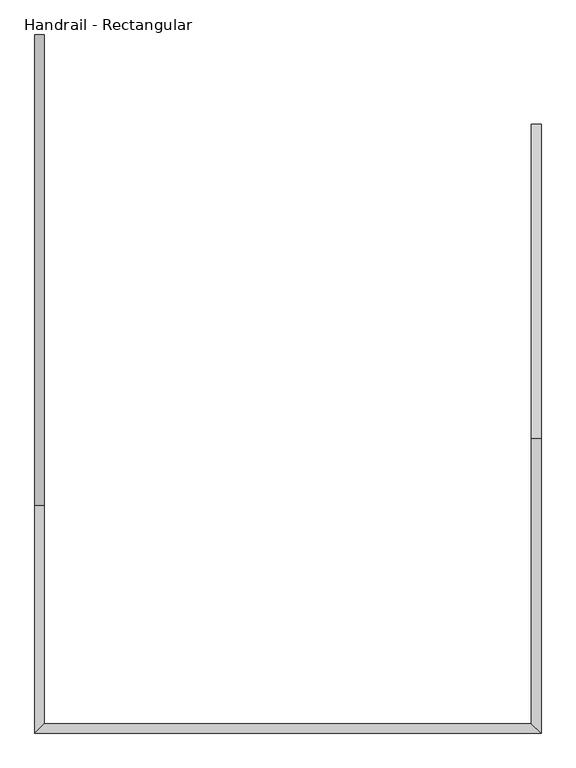
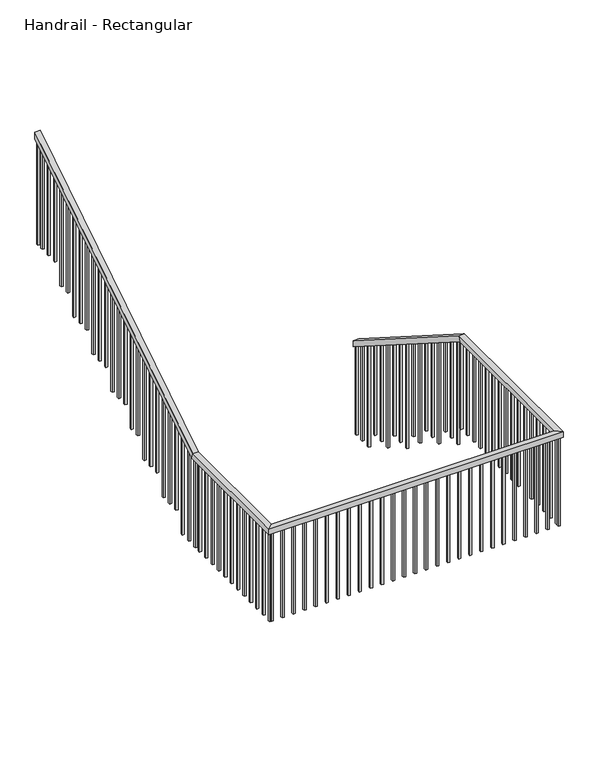
"""IFC4 building model written with IfcOpenShell, lengths in millimetres: railing geometry, Handrail - Rectangular."""

from ifc_helpers import new_model, si_unit, frame, origin, place, context, project, spatial, polyline, outline, extrude, faceted_brep, source, transform, mapped, element, save


def handrail_rectangular_a87038dc(model_context):
    return source(origin(), model_context, "Body", "SolidModel", [
        faceted_brep([(-73285.35, 12128.5, 20345.4), (-73285.35, 12128.5, 20285.186276), (-73336.15, 12128.5, 20285.186276), (-73336.15, 12128.5, 20345.4), (-73285.35, 10452.1, 21412.2), (-73285.35, 10437.3070051, 21361.4), (-73336.15, 10437.3070051, 21361.4), (-73336.15, 10452.1, 21412.2), (-73285.35, 8877.3, 21412.2), (-73285.35, 8877.3, 21361.4), (-73336.15, 8928.1, 21361.4), (-73336.15, 8928.1, 21412.2), (-75990.45, 8877.3, 21412.2), (-75990.45, 8877.3, 21361.4), (-75939.65, 8928.1, 21361.4), (-75939.65, 8928.1, 21412.2), (-75990.45, 10090.15, 21412.2), (-75990.45, 10104.9429949, 21361.4), (-75939.65, 10104.9429949, 21361.4), (-75939.65, 10090.15, 21412.2), (-75990.45, 12604.75, 23012.4), (-75939.65, 12604.75, 23012.4), (-75939.65, 12604.75, 22952.186276), (-75990.45, 12604.75, 22952.186276)], [[[0, 1, 2, 3]], [[1, 0, 4, 5]], [[2, 1, 5, 6]], [[3, 2, 6, 7]], [[0, 3, 7, 4]], [[5, 4, 8, 9]], [[6, 5, 9, 10]], [[7, 6, 10, 11]], [[4, 7, 11, 8]], [[9, 8, 12, 13]], [[10, 9, 13, 14]], [[11, 10, 14, 15]], [[8, 11, 15, 12]], [[13, 12, 16, 17]], [[14, 13, 17, 18]], [[15, 14, 18, 19]], [[12, 15, 19, 16]], [[20, 21, 22, 23]], [[17, 16, 20, 23]], [[18, 17, 23, 22]], [[19, 18, 22, 21]], [[16, 19, 21, 20]]]),
        extrude(outline(polyline([(12538.075, 22909.7567305), (12538.075, 21920.2), (12519.025, 21920.2), (12519.025, 22897.6340032), (12538.075, 22909.7567305)])), frame((-75974.575, 0.0, 0.0), z_axis=(1.0, 0.0, 0.0), x_axis=(0.0, 1.0, 0.0)), (0.0, 0.0, 1.0), 19.05),
        extrude(outline(polyline([(12436.475, 22845.1021851), (12436.475, 21920.2), (12417.425, 21920.2), (12417.425, 22832.9794578), (12436.475, 22845.1021851)])), frame((-75974.575, 0.0, 0.0), z_axis=(1.0, 0.0, 0.0), x_axis=(0.0, 1.0, 0.0)), (0.0, 0.0, 1.0), 19.05),
        extrude(outline(polyline([(12334.875, 22780.4476396), (12334.875, 21920.2), (12315.825, 21920.2), (12315.825, 22768.3249123), (12334.875, 22780.4476396)])), frame((-75974.575, 0.0, 0.0), z_axis=(1.0, 0.0, 0.0), x_axis=(0.0, 1.0, 0.0)), (0.0, 0.0, 1.0), 19.05),
        extrude(outline(polyline([(12233.275, 22715.7930941), (12233.275, 21742.4), (12214.225, 21742.4), (12214.225, 22703.6703669), (12233.275, 22715.7930941)])), frame((-75974.575, 0.0, 0.0), z_axis=(1.0, 0.0, 0.0), x_axis=(0.0, 1.0, 0.0)), (0.0, 0.0, 1.0), 19.05),
        extrude(outline(polyline([(12131.675, 22651.1385487), (12131.675, 21742.4), (12112.625, 21742.4), (12112.625, 22639.0158214), (12131.675, 22651.1385487)])), frame((-75974.575, 0.0, 0.0), z_axis=(1.0, 0.0, 0.0), x_axis=(0.0, 1.0, 0.0)), (0.0, 0.0, 1.0), 19.05),
        extrude(outline(polyline([(12030.075, 22586.4840032), (12030.075, 21564.6), (12011.025, 21564.6), (12011.025, 22574.361276), (12030.075, 22586.4840032)])), frame((-75974.575, 0.0, 0.0), z_axis=(1.0, 0.0, 0.0), x_axis=(0.0, 1.0, 0.0)), (0.0, 0.0, 1.0), 19.05),
        extrude(outline(polyline([(11928.475, 22521.8294578), (11928.475, 21564.6), (11909.425, 21564.6), (11909.425, 22509.7067305), (11928.475, 22521.8294578)])), frame((-75974.575, 0.0, 0.0), z_axis=(1.0, 0.0, 0.0), x_axis=(0.0, 1.0, 0.0)), (0.0, 0.0, 1.0), 19.05),
        extrude(outline(polyline([(11826.875, 22457.1749123), (11826.875, 21564.6), (11807.825, 21564.6), (11807.825, 22445.0521851), (11826.875, 22457.1749123)])), frame((-75974.575, 0.0, 0.0), z_axis=(1.0, 0.0, 0.0), x_axis=(0.0, 1.0, 0.0)), (0.0, 0.0, 1.0), 19.05),
        extrude(outline(polyline([(11725.275, 22392.5203669), (11725.275, 21386.8), (11706.225, 21386.8), (11706.225, 22380.3976396), (11725.275, 22392.5203669)])), frame((-75974.575, 0.0, 0.0), z_axis=(1.0, 0.0, 0.0), x_axis=(0.0, 1.0, 0.0)), (0.0, 0.0, 1.0), 19.05),
        extrude(outline(polyline([(11623.675, 22327.8658214), (11623.675, 21386.8), (11604.625, 21386.8), (11604.625, 22315.7430941), (11623.675, 22327.8658214)])), frame((-75974.575, 0.0, 0.0), z_axis=(1.0, 0.0, 0.0), x_axis=(0.0, 1.0, 0.0)), (0.0, 0.0, 1.0), 19.05),
        extrude(outline(polyline([(11522.075, 22263.211276), (11522.075, 21386.8), (11503.025, 21386.8), (11503.025, 22251.0885487), (11522.075, 22263.211276)])), frame((-75974.575, 0.0, 0.0), z_axis=(1.0, 0.0, 0.0), x_axis=(0.0, 1.0, 0.0)), (0.0, 0.0, 1.0), 19.05),
        extrude(outline(polyline([(11420.475, 22198.5567305), (11420.475, 21209.0), (11401.425, 21209.0), (11401.425, 22186.4340032), (11420.475, 22198.5567305)])), frame((-75974.575, 0.0, 0.0), z_axis=(1.0, 0.0, 0.0), x_axis=(0.0, 1.0, 0.0)), (0.0, 0.0, 1.0), 19.05),
        extrude(outline(polyline([(11318.875, 22133.9021851), (11318.875, 21209.0), (11299.825, 21209.0), (11299.825, 22121.7794578), (11318.875, 22133.9021851)])), frame((-75974.575, 0.0, 0.0), z_axis=(1.0, 0.0, 0.0), x_axis=(0.0, 1.0, 0.0)), (0.0, 0.0, 1.0), 19.05),
        extrude(outline(polyline([(11217.275, 22069.2476396), (11217.275, 21209.0), (11198.225, 21209.0), (11198.225, 22057.1249123), (11217.275, 22069.2476396)])), frame((-75974.575, 0.0, 0.0), z_axis=(1.0, 0.0, 0.0), x_axis=(0.0, 1.0, 0.0)), (0.0, 0.0, 1.0), 19.05),
        extrude(outline(polyline([(11115.675, 22004.5930941), (11115.675, 21031.2), (11096.625, 21031.2), (11096.625, 21992.4703669), (11115.675, 22004.5930941)])), frame((-75974.575, 0.0, 0.0), z_axis=(1.0, 0.0, 0.0), x_axis=(0.0, 1.0, 0.0)), (0.0, 0.0, 1.0), 19.05),
        extrude(outline(polyline([(11014.075, 21939.9385487), (11014.075, 21031.2), (10995.025, 21031.2), (10995.025, 21927.8158214), (11014.075, 21939.9385487)])), frame((-75974.575, 0.0, 0.0), z_axis=(1.0, 0.0, 0.0), x_axis=(0.0, 1.0, 0.0)), (0.0, 0.0, 1.0), 19.05),
        extrude(outline(polyline([(10912.475, 21875.2840032), (10912.475, 20853.4), (10893.425, 20853.4), (10893.425, 21863.161276), (10912.475, 21875.2840032)])), frame((-75974.575, 0.0, 0.0), z_axis=(1.0, 0.0, 0.0), x_axis=(0.0, 1.0, 0.0)), (0.0, 0.0, 1.0), 19.05),
        extrude(outline(polyline([(10810.875, 21810.6294578), (10810.875, 20853.4), (10791.825, 20853.4), (10791.825, 21798.5067305), (10810.875, 21810.6294578)])), frame((-75974.575, 0.0, 0.0), z_axis=(1.0, 0.0, 0.0), x_axis=(0.0, 1.0, 0.0)), (0.0, 0.0, 1.0), 19.05),
        extrude(outline(polyline([(10709.275, 21745.9749123), (10709.275, 20853.4), (10690.225, 20853.4), (10690.225, 21733.8521851), (10709.275, 21745.9749123)])), frame((-75974.575, 0.0, 0.0), z_axis=(1.0, 0.0, 0.0), x_axis=(0.0, 1.0, 0.0)), (0.0, 0.0, 1.0), 19.05),
        extrude(outline(polyline([(10607.675, 21681.3203669), (10607.675, 20675.6), (10588.625, 20675.6), (10588.625, 21669.1976396), (10607.675, 21681.3203669)])), frame((-75974.575, 0.0, 0.0), z_axis=(1.0, 0.0, 0.0), x_axis=(0.0, 1.0, 0.0)), (0.0, 0.0, 1.0), 19.05),
        extrude(outline(polyline([(10506.075, 21616.6658214), (10506.075, 20675.6), (10487.025, 20675.6), (10487.025, 21604.5430941), (10506.075, 21616.6658214)])), frame((-75974.575, 0.0, 0.0), z_axis=(1.0, 0.0, 0.0), x_axis=(0.0, 1.0, 0.0)), (0.0, 0.0, 1.0), 19.05),
        extrude(outline(polyline([(10404.475, 21552.011276), (10404.475, 20675.6), (10385.425, 20675.6), (10385.425, 21539.8885487), (10404.475, 21552.011276)])), frame((-75974.575, 0.0, 0.0), z_axis=(1.0, 0.0, 0.0), x_axis=(0.0, 1.0, 0.0)), (0.0, 0.0, 1.0), 19.05),
        extrude(outline(polyline([(10302.875, 21487.3567305), (10302.875, 20497.8), (10283.825, 20497.8), (10283.825, 21475.2340032), (10302.875, 21487.3567305)])), frame((-75974.575, 0.0, 0.0), z_axis=(1.0, 0.0, 0.0), x_axis=(0.0, 1.0, 0.0)), (0.0, 0.0, 1.0), 19.05),
        extrude(outline(polyline([(10201.275, 21422.7021851), (10201.275, 20497.8), (10182.225, 20497.8), (10182.225, 21410.5794578), (10201.275, 21422.7021851)])), frame((-75974.575, 0.0, 0.0), z_axis=(1.0, 0.0, 0.0), x_axis=(0.0, 1.0, 0.0)), (0.0, 0.0, 1.0), 19.05),
        extrude(outline(polyline([(-75974.575, 10010.775), (-75974.575, 10029.825), (-75955.525, 10029.825), (-75955.525, 10010.775), (-75974.575, 10010.775)])), frame((0.0, 0.0, 20497.8), z_axis=(0.0, 0.0, 1.0), x_axis=(1.0, 0.0, 0.0)), (0.0, 0.0, 1.0), 863.6),
        extrude(outline(polyline([(-75974.575, 9909.175), (-75974.575, 9928.225), (-75955.525, 9928.225), (-75955.525, 9909.175), (-75974.575, 9909.175)])), frame((0.0, 0.0, 20497.8), z_axis=(0.0, 0.0, 1.0), x_axis=(1.0, 0.0, 0.0)), (0.0, 0.0, 1.0), 863.6),
        extrude(outline(polyline([(-75974.575, 9807.575), (-75974.575, 9826.625), (-75955.525, 9826.625), (-75955.525, 9807.575), (-75974.575, 9807.575)])), frame((0.0, 0.0, 20497.8), z_axis=(0.0, 0.0, 1.0), x_axis=(1.0, 0.0, 0.0)), (0.0, 0.0, 1.0), 863.6),
        extrude(outline(polyline([(-75974.575, 9705.975), (-75974.575, 9725.025), (-75955.525, 9725.025), (-75955.525, 9705.975), (-75974.575, 9705.975)])), frame((0.0, 0.0, 20497.8), z_axis=(0.0, 0.0, 1.0), x_axis=(1.0, 0.0, 0.0)), (0.0, 0.0, 1.0), 863.6),
        extrude(outline(polyline([(-75974.575, 9604.375), (-75974.575, 9623.425), (-75955.525, 9623.425), (-75955.525, 9604.375), (-75974.575, 9604.375)])), frame((0.0, 0.0, 20497.8), z_axis=(0.0, 0.0, 1.0), x_axis=(1.0, 0.0, 0.0)), (0.0, 0.0, 1.0), 863.6),
        extrude(outline(polyline([(-75974.575, 9502.775), (-75974.575, 9521.825), (-75955.525, 9521.825), (-75955.525, 9502.775), (-75974.575, 9502.775)])), frame((0.0, 0.0, 20497.8), z_axis=(0.0, 0.0, 1.0), x_axis=(1.0, 0.0, 0.0)), (0.0, 0.0, 1.0), 863.6),
        extrude(outline(polyline([(-75974.575, 9401.175), (-75974.575, 9420.225), (-75955.525, 9420.225), (-75955.525, 9401.175), (-75974.575, 9401.175)])), frame((0.0, 0.0, 20497.8), z_axis=(0.0, 0.0, 1.0), x_axis=(1.0, 0.0, 0.0)), (0.0, 0.0, 1.0), 863.6),
        extrude(outline(polyline([(-75974.575, 9299.575), (-75974.575, 9318.625), (-75955.525, 9318.625), (-75955.525, 9299.575), (-75974.575, 9299.575)])), frame((0.0, 0.0, 20497.8), z_axis=(0.0, 0.0, 1.0), x_axis=(1.0, 0.0, 0.0)), (0.0, 0.0, 1.0), 863.6),
        extrude(outline(polyline([(-75974.575, 9197.975), (-75974.575, 9217.025), (-75955.525, 9217.025), (-75955.525, 9197.975), (-75974.575, 9197.975)])), frame((0.0, 0.0, 20497.8), z_axis=(0.0, 0.0, 1.0), x_axis=(1.0, 0.0, 0.0)), (0.0, 0.0, 1.0), 863.6),
        extrude(outline(polyline([(-75974.575, 9096.375), (-75974.575, 9115.425), (-75955.525, 9115.425), (-75955.525, 9096.375), (-75974.575, 9096.375)])), frame((0.0, 0.0, 20497.8), z_axis=(0.0, 0.0, 1.0), x_axis=(1.0, 0.0, 0.0)), (0.0, 0.0, 1.0), 863.6),
        extrude(outline(polyline([(-75974.575, 8994.775), (-75974.575, 9013.825), (-75955.525, 9013.825), (-75955.525, 8994.775), (-75974.575, 8994.775)])), frame((0.0, 0.0, 20497.8), z_axis=(0.0, 0.0, 1.0), x_axis=(1.0, 0.0, 0.0)), (0.0, 0.0, 1.0), 863.6),
        extrude(outline(polyline([(-75942.825, 8893.175), (-75961.875, 8893.175), (-75961.875, 8912.225), (-75942.825, 8912.225), (-75942.825, 8893.175)])), frame((0.0, 0.0, 20497.8), z_axis=(0.0, 0.0, 1.0), x_axis=(1.0, 0.0, 0.0)), (0.0, 0.0, 1.0), 863.6),
        extrude(outline(polyline([(-75841.225, 8893.175), (-75860.275, 8893.175), (-75860.275, 8912.225), (-75841.225, 8912.225), (-75841.225, 8893.175)])), frame((0.0, 0.0, 20497.8), z_axis=(0.0, 0.0, 1.0), x_axis=(1.0, 0.0, 0.0)), (0.0, 0.0, 1.0), 863.6),
        extrude(outline(polyline([(-75739.625, 8893.175), (-75758.675, 8893.175), (-75758.675, 8912.225), (-75739.625, 8912.225), (-75739.625, 8893.175)])), frame((0.0, 0.0, 20497.8), z_axis=(0.0, 0.0, 1.0), x_axis=(1.0, 0.0, 0.0)), (0.0, 0.0, 1.0), 863.6),
        extrude(outline(polyline([(-75638.025, 8893.175), (-75657.075, 8893.175), (-75657.075, 8912.225), (-75638.025, 8912.225), (-75638.025, 8893.175)])), frame((0.0, 0.0, 20497.8), z_axis=(0.0, 0.0, 1.0), x_axis=(1.0, 0.0, 0.0)), (0.0, 0.0, 1.0), 863.6),
        extrude(outline(polyline([(-75536.425, 8893.175), (-75555.475, 8893.175), (-75555.475, 8912.225), (-75536.425, 8912.225), (-75536.425, 8893.175)])), frame((0.0, 0.0, 20497.8), z_axis=(0.0, 0.0, 1.0), x_axis=(1.0, 0.0, 0.0)), (0.0, 0.0, 1.0), 863.6),
        extrude(outline(polyline([(-75434.825, 8893.175), (-75453.875, 8893.175), (-75453.875, 8912.225), (-75434.825, 8912.225), (-75434.825, 8893.175)])), frame((0.0, 0.0, 20497.8), z_axis=(0.0, 0.0, 1.0), x_axis=(1.0, 0.0, 0.0)), (0.0, 0.0, 1.0), 863.6),
        extrude(outline(polyline([(-75333.225, 8893.175), (-75352.275, 8893.175), (-75352.275, 8912.225), (-75333.225, 8912.225), (-75333.225, 8893.175)])), frame((0.0, 0.0, 20497.8), z_axis=(0.0, 0.0, 1.0), x_axis=(1.0, 0.0, 0.0)), (0.0, 0.0, 1.0), 863.6),
        extrude(outline(polyline([(-75231.625, 8893.175), (-75250.675, 8893.175), (-75250.675, 8912.225), (-75231.625, 8912.225), (-75231.625, 8893.175)])), frame((0.0, 0.0, 20497.8), z_axis=(0.0, 0.0, 1.0), x_axis=(1.0, 0.0, 0.0)), (0.0, 0.0, 1.0), 863.6),
        extrude(outline(polyline([(-75130.025, 8893.175), (-75149.075, 8893.175), (-75149.075, 8912.225), (-75130.025, 8912.225), (-75130.025, 8893.175)])), frame((0.0, 0.0, 20497.8), z_axis=(0.0, 0.0, 1.0), x_axis=(1.0, 0.0, 0.0)), (0.0, 0.0, 1.0), 863.6),
        extrude(outline(polyline([(-75028.425, 8893.175), (-75047.475, 8893.175), (-75047.475, 8912.225), (-75028.425, 8912.225), (-75028.425, 8893.175)])), frame((0.0, 0.0, 20497.8), z_axis=(0.0, 0.0, 1.0), x_axis=(1.0, 0.0, 0.0)), (0.0, 0.0, 1.0), 863.6),
        extrude(outline(polyline([(-74926.825, 8893.175), (-74945.875, 8893.175), (-74945.875, 8912.225), (-74926.825, 8912.225), (-74926.825, 8893.175)])), frame((0.0, 0.0, 20497.8), z_axis=(0.0, 0.0, 1.0), x_axis=(1.0, 0.0, 0.0)), (0.0, 0.0, 1.0), 863.6),
        extrude(outline(polyline([(-74825.225, 8893.175), (-74844.275, 8893.175), (-74844.275, 8912.225), (-74825.225, 8912.225), (-74825.225, 8893.175)])), frame((0.0, 0.0, 20497.8), z_axis=(0.0, 0.0, 1.0), x_axis=(1.0, 0.0, 0.0)), (0.0, 0.0, 1.0), 863.6),
        extrude(outline(polyline([(-74723.625, 8893.175), (-74742.675, 8893.175), (-74742.675, 8912.225), (-74723.625, 8912.225), (-74723.625, 8893.175)])), frame((0.0, 0.0, 20497.8), z_axis=(0.0, 0.0, 1.0), x_axis=(1.0, 0.0, 0.0)), (0.0, 0.0, 1.0), 863.6),
        extrude(outline(polyline([(-74622.025, 8893.175), (-74641.075, 8893.175), (-74641.075, 8912.225), (-74622.025, 8912.225), (-74622.025, 8893.175)])), frame((0.0, 0.0, 20497.8), z_axis=(0.0, 0.0, 1.0), x_axis=(1.0, 0.0, 0.0)), (0.0, 0.0, 1.0), 863.6),
        extrude(outline(polyline([(-74520.425, 8893.175), (-74539.475, 8893.175), (-74539.475, 8912.225), (-74520.425, 8912.225), (-74520.425, 8893.175)])), frame((0.0, 0.0, 20497.8), z_axis=(0.0, 0.0, 1.0), x_axis=(1.0, 0.0, 0.0)), (0.0, 0.0, 1.0), 863.6),
        extrude(outline(polyline([(-74418.825, 8893.175), (-74437.875, 8893.175), (-74437.875, 8912.225), (-74418.825, 8912.225), (-74418.825, 8893.175)])), frame((0.0, 0.0, 20497.8), z_axis=(0.0, 0.0, 1.0), x_axis=(1.0, 0.0, 0.0)), (0.0, 0.0, 1.0), 863.6),
        extrude(outline(polyline([(-74317.225, 8893.175), (-74336.275, 8893.175), (-74336.275, 8912.225), (-74317.225, 8912.225), (-74317.225, 8893.175)])), frame((0.0, 0.0, 20497.8), z_axis=(0.0, 0.0, 1.0), x_axis=(1.0, 0.0, 0.0)), (0.0, 0.0, 1.0), 863.6),
        extrude(outline(polyline([(-74215.625, 8893.175), (-74234.675, 8893.175), (-74234.675, 8912.225), (-74215.625, 8912.225), (-74215.625, 8893.175)])), frame((0.0, 0.0, 20497.8), z_axis=(0.0, 0.0, 1.0), x_axis=(1.0, 0.0, 0.0)), (0.0, 0.0, 1.0), 863.6),
        extrude(outline(polyline([(-74114.025, 8893.175), (-74133.075, 8893.175), (-74133.075, 8912.225), (-74114.025, 8912.225), (-74114.025, 8893.175)])), frame((0.0, 0.0, 20497.8), z_axis=(0.0, 0.0, 1.0), x_axis=(1.0, 0.0, 0.0)), (0.0, 0.0, 1.0), 863.6),
        extrude(outline(polyline([(-74012.425, 8893.175), (-74031.475, 8893.175), (-74031.475, 8912.225), (-74012.425, 8912.225), (-74012.425, 8893.175)])), frame((0.0, 0.0, 20497.8), z_axis=(0.0, 0.0, 1.0), x_axis=(1.0, 0.0, 0.0)), (0.0, 0.0, 1.0), 863.6),
        extrude(outline(polyline([(-73910.825, 8893.175), (-73929.875, 8893.175), (-73929.875, 8912.225), (-73910.825, 8912.225), (-73910.825, 8893.175)])), frame((0.0, 0.0, 20497.8), z_axis=(0.0, 0.0, 1.0), x_axis=(1.0, 0.0, 0.0)), (0.0, 0.0, 1.0), 863.6),
        extrude(outline(polyline([(-73809.225, 8893.175), (-73828.275, 8893.175), (-73828.275, 8912.225), (-73809.225, 8912.225), (-73809.225, 8893.175)])), frame((0.0, 0.0, 20497.8), z_axis=(0.0, 0.0, 1.0), x_axis=(1.0, 0.0, 0.0)), (0.0, 0.0, 1.0), 863.6),
        extrude(outline(polyline([(-73707.625, 8893.175), (-73726.675, 8893.175), (-73726.675, 8912.225), (-73707.625, 8912.225), (-73707.625, 8893.175)])), frame((0.0, 0.0, 20497.8), z_axis=(0.0, 0.0, 1.0), x_axis=(1.0, 0.0, 0.0)), (0.0, 0.0, 1.0), 863.6),
        extrude(outline(polyline([(-73606.025, 8893.175), (-73625.075, 8893.175), (-73625.075, 8912.225), (-73606.025, 8912.225), (-73606.025, 8893.175)])), frame((0.0, 0.0, 20497.8), z_axis=(0.0, 0.0, 1.0), x_axis=(1.0, 0.0, 0.0)), (0.0, 0.0, 1.0), 863.6),
        extrude(outline(polyline([(-73504.425, 8893.175), (-73523.475, 8893.175), (-73523.475, 8912.225), (-73504.425, 8912.225), (-73504.425, 8893.175)])), frame((0.0, 0.0, 20497.8), z_axis=(0.0, 0.0, 1.0), x_axis=(1.0, 0.0, 0.0)), (0.0, 0.0, 1.0), 863.6),
        extrude(outline(polyline([(-73402.825, 8893.175), (-73421.875, 8893.175), (-73421.875, 8912.225), (-73402.825, 8912.225), (-73402.825, 8893.175)])), frame((0.0, 0.0, 20497.8), z_axis=(0.0, 0.0, 1.0), x_axis=(1.0, 0.0, 0.0)), (0.0, 0.0, 1.0), 863.6),
        extrude(outline(polyline([(-73301.225, 8937.625), (-73301.225, 8918.575), (-73320.275, 8918.575), (-73320.275, 8937.625), (-73301.225, 8937.625)])), frame((0.0, 0.0, 20497.8), z_axis=(0.0, 0.0, 1.0), x_axis=(1.0, 0.0, 0.0)), (0.0, 0.0, 1.0), 863.6),
        extrude(outline(polyline([(-73301.225, 9039.225), (-73301.225, 9020.175), (-73320.275, 9020.175), (-73320.275, 9039.225), (-73301.225, 9039.225)])), frame((0.0, 0.0, 20497.8), z_axis=(0.0, 0.0, 1.0), x_axis=(1.0, 0.0, 0.0)), (0.0, 0.0, 1.0), 863.6),
        extrude(outline(polyline([(-73301.225, 9140.825), (-73301.225, 9121.775), (-73320.275, 9121.775), (-73320.275, 9140.825), (-73301.225, 9140.825)])), frame((0.0, 0.0, 20497.8), z_axis=(0.0, 0.0, 1.0), x_axis=(1.0, 0.0, 0.0)), (0.0, 0.0, 1.0), 863.6),
        extrude(outline(polyline([(-73301.225, 9242.425), (-73301.225, 9223.375), (-73320.275, 9223.375), (-73320.275, 9242.425), (-73301.225, 9242.425)])), frame((0.0, 0.0, 20497.8), z_axis=(0.0, 0.0, 1.0), x_axis=(1.0, 0.0, 0.0)), (0.0, 0.0, 1.0), 863.6),
        extrude(outline(polyline([(-73301.225, 9344.025), (-73301.225, 9324.975), (-73320.275, 9324.975), (-73320.275, 9344.025), (-73301.225, 9344.025)])), frame((0.0, 0.0, 20497.8), z_axis=(0.0, 0.0, 1.0), x_axis=(1.0, 0.0, 0.0)), (0.0, 0.0, 1.0), 863.6),
        extrude(outline(polyline([(-73301.225, 9445.625), (-73301.225, 9426.575), (-73320.275, 9426.575), (-73320.275, 9445.625), (-73301.225, 9445.625)])), frame((0.0, 0.0, 20497.8), z_axis=(0.0, 0.0, 1.0), x_axis=(1.0, 0.0, 0.0)), (0.0, 0.0, 1.0), 863.6),
        extrude(outline(polyline([(-73301.225, 9547.225), (-73301.225, 9528.175), (-73320.275, 9528.175), (-73320.275, 9547.225), (-73301.225, 9547.225)])), frame((0.0, 0.0, 20497.8), z_axis=(0.0, 0.0, 1.0), x_axis=(1.0, 0.0, 0.0)), (0.0, 0.0, 1.0), 863.6),
        extrude(outline(polyline([(-73301.225, 9648.825), (-73301.225, 9629.775), (-73320.275, 9629.775), (-73320.275, 9648.825), (-73301.225, 9648.825)])), frame((0.0, 0.0, 20497.8), z_axis=(0.0, 0.0, 1.0), x_axis=(1.0, 0.0, 0.0)), (0.0, 0.0, 1.0), 863.6),
        extrude(outline(polyline([(-73301.225, 9750.425), (-73301.225, 9731.375), (-73320.275, 9731.375), (-73320.275, 9750.425), (-73301.225, 9750.425)])), frame((0.0, 0.0, 20497.8), z_axis=(0.0, 0.0, 1.0), x_axis=(1.0, 0.0, 0.0)), (0.0, 0.0, 1.0), 863.6),
        extrude(outline(polyline([(-73301.225, 9852.025), (-73301.225, 9832.975), (-73320.275, 9832.975), (-73320.275, 9852.025), (-73301.225, 9852.025)])), frame((0.0, 0.0, 20497.8), z_axis=(0.0, 0.0, 1.0), x_axis=(1.0, 0.0, 0.0)), (0.0, 0.0, 1.0), 863.6),
        extrude(outline(polyline([(-73301.225, 9953.625), (-73301.225, 9934.575), (-73320.275, 9934.575), (-73320.275, 9953.625), (-73301.225, 9953.625)])), frame((0.0, 0.0, 20497.8), z_axis=(0.0, 0.0, 1.0), x_axis=(1.0, 0.0, 0.0)), (0.0, 0.0, 1.0), 863.6),
        extrude(outline(polyline([(-73301.225, 10055.225), (-73301.225, 10036.175), (-73320.275, 10036.175), (-73320.275, 10055.225), (-73301.225, 10055.225)])), frame((0.0, 0.0, 20497.8), z_axis=(0.0, 0.0, 1.0), x_axis=(1.0, 0.0, 0.0)), (0.0, 0.0, 1.0), 863.6),
        extrude(outline(polyline([(-73301.225, 10156.825), (-73301.225, 10137.775), (-73320.275, 10137.775), (-73320.275, 10156.825), (-73301.225, 10156.825)])), frame((0.0, 0.0, 20497.8), z_axis=(0.0, 0.0, 1.0), x_axis=(1.0, 0.0, 0.0)), (0.0, 0.0, 1.0), 863.6),
        extrude(outline(polyline([(-73301.225, 10258.425), (-73301.225, 10239.375), (-73320.275, 10239.375), (-73320.275, 10258.425), (-73301.225, 10258.425)])), frame((0.0, 0.0, 20497.8), z_axis=(0.0, 0.0, 1.0), x_axis=(1.0, 0.0, 0.0)), (0.0, 0.0, 1.0), 863.6),
        extrude(outline(polyline([(-73301.225, 10360.025), (-73301.225, 10340.975), (-73320.275, 10340.975), (-73320.275, 10360.025), (-73301.225, 10360.025)])), frame((0.0, 0.0, 20497.8), z_axis=(0.0, 0.0, 1.0), x_axis=(1.0, 0.0, 0.0)), (0.0, 0.0, 1.0), 863.6),
        extrude(outline(polyline([(10512.425, 21313.5976396), (10512.425, 20320.0), (10493.375, 20320.0), (10493.375, 21325.7203669), (10512.425, 21313.5976396)])), frame((-73320.275, 0.0, 0.0), z_axis=(1.0, 0.0, 0.0), x_axis=(0.0, 1.0, 0.0)), (0.0, 0.0, 1.0), 19.05),
        extrude(outline(polyline([(10614.025, 21248.9430941), (10614.025, 20320.0), (10594.975, 20320.0), (10594.975, 21261.0658214), (10614.025, 21248.9430941)])), frame((-73320.275, 0.0, 0.0), z_axis=(1.0, 0.0, 0.0), x_axis=(0.0, 1.0, 0.0)), (0.0, 0.0, 1.0), 19.05),
        extrude(outline(polyline([(10715.625, 21184.2885487), (10715.625, 20320.0), (10696.575, 20320.0), (10696.575, 21196.411276), (10715.625, 21184.2885487)])), frame((-73320.275, 0.0, 0.0), z_axis=(1.0, 0.0, 0.0), x_axis=(0.0, 1.0, 0.0)), (0.0, 0.0, 1.0), 19.05),
        extrude(outline(polyline([(10817.225, 21119.6340032), (10817.225, 20142.2), (10798.175, 20142.2), (10798.175, 21131.7567305), (10817.225, 21119.6340032)])), frame((-73320.275, 0.0, 0.0), z_axis=(1.0, 0.0, 0.0), x_axis=(0.0, 1.0, 0.0)), (0.0, 0.0, 1.0), 19.05),
        extrude(outline(polyline([(10918.825, 21054.9794578), (10918.825, 20142.2), (10899.775, 20142.2), (10899.775, 21067.1021851), (10918.825, 21054.9794578)])), frame((-73320.275, 0.0, 0.0), z_axis=(1.0, 0.0, 0.0), x_axis=(0.0, 1.0, 0.0)), (0.0, 0.0, 1.0), 19.05),
        extrude(outline(polyline([(11020.425, 20990.3249123), (11020.425, 20142.2), (11001.375, 20142.2), (11001.375, 21002.4476396), (11020.425, 20990.3249123)])), frame((-73320.275, 0.0, 0.0), z_axis=(1.0, 0.0, 0.0), x_axis=(0.0, 1.0, 0.0)), (0.0, 0.0, 1.0), 19.05),
        extrude(outline(polyline([(11122.025, 20925.6703669), (11122.025, 19964.4), (11102.975, 19964.4), (11102.975, 20937.7930941), (11122.025, 20925.6703669)])), frame((-73320.275, 0.0, 0.0), z_axis=(1.0, 0.0, 0.0), x_axis=(0.0, 1.0, 0.0)), (0.0, 0.0, 1.0), 19.05),
        extrude(outline(polyline([(11223.625, 20861.0158214), (11223.625, 19964.4), (11204.575, 19964.4), (11204.575, 20873.1385487), (11223.625, 20861.0158214)])), frame((-73320.275, 0.0, 0.0), z_axis=(1.0, 0.0, 0.0), x_axis=(0.0, 1.0, 0.0)), (0.0, 0.0, 1.0), 19.05),
        extrude(outline(polyline([(11325.225, 20796.361276), (11325.225, 19786.6), (11306.175, 19786.6), (11306.175, 20808.4840032), (11325.225, 20796.361276)])), frame((-73320.275, 0.0, 0.0), z_axis=(1.0, 0.0, 0.0), x_axis=(0.0, 1.0, 0.0)), (0.0, 0.0, 1.0), 19.05),
        extrude(outline(polyline([(11426.825, 20731.7067305), (11426.825, 19786.6), (11407.775, 19786.6), (11407.775, 20743.8294578), (11426.825, 20731.7067305)])), frame((-73320.275, 0.0, 0.0), z_axis=(1.0, 0.0, 0.0), x_axis=(0.0, 1.0, 0.0)), (0.0, 0.0, 1.0), 19.05),
        extrude(outline(polyline([(11528.425, 20667.0521851), (11528.425, 19786.6), (11509.375, 19786.6), (11509.375, 20679.1749123), (11528.425, 20667.0521851)])), frame((-73320.275, 0.0, 0.0), z_axis=(1.0, 0.0, 0.0), x_axis=(0.0, 1.0, 0.0)), (0.0, 0.0, 1.0), 19.05),
        extrude(outline(polyline([(11630.025, 20602.3976396), (11630.025, 19608.8), (11610.975, 19608.8), (11610.975, 20614.5203669), (11630.025, 20602.3976396)])), frame((-73320.275, 0.0, 0.0), z_axis=(1.0, 0.0, 0.0), x_axis=(0.0, 1.0, 0.0)), (0.0, 0.0, 1.0), 19.05),
        extrude(outline(polyline([(11731.625, 20537.7430941), (11731.625, 19608.8), (11712.575, 19608.8), (11712.575, 20549.8658214), (11731.625, 20537.7430941)])), frame((-73320.275, 0.0, 0.0), z_axis=(1.0, 0.0, 0.0), x_axis=(0.0, 1.0, 0.0)), (0.0, 0.0, 1.0), 19.05),
        extrude(outline(polyline([(11833.225, 20473.0885487), (11833.225, 19608.8), (11814.175, 19608.8), (11814.175, 20485.211276), (11833.225, 20473.0885487)])), frame((-73320.275, 0.0, 0.0), z_axis=(1.0, 0.0, 0.0), x_axis=(0.0, 1.0, 0.0)), (0.0, 0.0, 1.0), 19.05),
        extrude(outline(polyline([(11934.825, 20408.4340032), (11934.825, 19431.0), (11915.775, 19431.0), (11915.775, 20420.5567305), (11934.825, 20408.4340032)])), frame((-73320.275, 0.0, 0.0), z_axis=(1.0, 0.0, 0.0), x_axis=(0.0, 1.0, 0.0)), (0.0, 0.0, 1.0), 19.05),
        extrude(outline(polyline([(12036.425, 20343.7794578), (12036.425, 19431.0), (12017.375, 19431.0), (12017.375, 20355.9021851), (12036.425, 20343.7794578)])), frame((-73320.275, 0.0, 0.0), z_axis=(1.0, 0.0, 0.0), x_axis=(0.0, 1.0, 0.0)), (0.0, 0.0, 1.0), 19.05),
        extrude(outline(polyline([(-75974.575, 10080.625), (-75974.575, 10099.675), (-75955.525, 10099.675), (-75955.525, 10080.625), (-75974.575, 10080.625)])), frame((0.0, 0.0, 20497.8), z_axis=(0.0, 0.0, 1.0), x_axis=(1.0, 0.0, 0.0)), (0.0, 0.0, 1.0), 863.6),
        extrude(outline(polyline([(-75955.525, 8893.175), (-75974.575, 8893.175), (-75974.575, 8912.225), (-75955.525, 8912.225), (-75955.525, 8893.175)])), frame((0.0, 0.0, 20497.8), z_axis=(0.0, 0.0, 1.0), x_axis=(1.0, 0.0, 0.0)), (0.0, 0.0, 1.0), 863.6),
        extrude(outline(polyline([(-73301.225, 8912.225), (-73301.225, 8893.175), (-73320.275, 8893.175), (-73320.275, 8912.225), (-73301.225, 8912.225)])), frame((0.0, 0.0, 20497.8), z_axis=(0.0, 0.0, 1.0), x_axis=(1.0, 0.0, 0.0)), (0.0, 0.0, 1.0), 863.6),
        extrude(outline(polyline([(10461.625, 21345.9249123), (10461.625, 20497.8), (10442.575, 20497.8), (10442.575, 21358.0476396), (10461.625, 21345.9249123)])), frame((-73320.275, 0.0, 0.0), z_axis=(1.0, 0.0, 0.0), x_axis=(0.0, 1.0, 0.0)), (0.0, 0.0, 1.0), 19.05),
        extrude(outline(polyline([(12604.75, 22952.186276), (12604.75, 21920.2), (12585.7, 21920.2), (12585.7, 22940.0635487), (12604.75, 22952.186276)])), frame((-75974.575, 0.0, 0.0), z_axis=(1.0, 0.0, 0.0), x_axis=(0.0, 1.0, 0.0)), (0.0, 0.0, 1.0), 19.05),
        extrude(outline(polyline([(12128.5, 20285.186276), (12128.5, 19431.0), (12109.45, 19431.0), (12109.45, 20297.3090032), (12128.5, 20285.186276)])), frame((-73320.275, 0.0, 0.0), z_axis=(1.0, 0.0, 0.0), x_axis=(0.0, 1.0, 0.0)), (0.0, 0.0, 1.0), 19.05),
    ])


if __name__ == "__main__":
    model = new_model("IFC4")
    model_context = context("Model", 3, world=origin())
    ifc_project = project(units=[si_unit("LENGTHUNIT", "METRE", prefix="MILLI")], contexts=[model_context])
    site = spatial("IfcSite", under=ifc_project)
    building = spatial("IfcBuilding", under=site)
    placement = place(None, origin())
    handrail_rectangular_shape = handrail_rectangular_a87038dc(model_context)
    element("IfcRailing", 1, ObjectType="Handrail - Rectangular", at=placement, inside=building, context=model_context, shape_type="MappedRepresentation", body=[
        mapped(handrail_rectangular_shape, transform((0.0, 0.0, 0.0), x_axis=(1.0, 0.0, 0.0), y_axis=(0.0, 1.0, 0.0), z_axis=(0.0, 0.0, 1.0))),
    ])
    save(model, "model.ifc")
